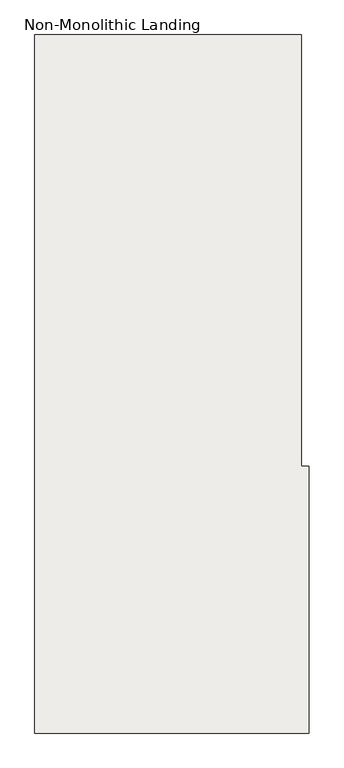
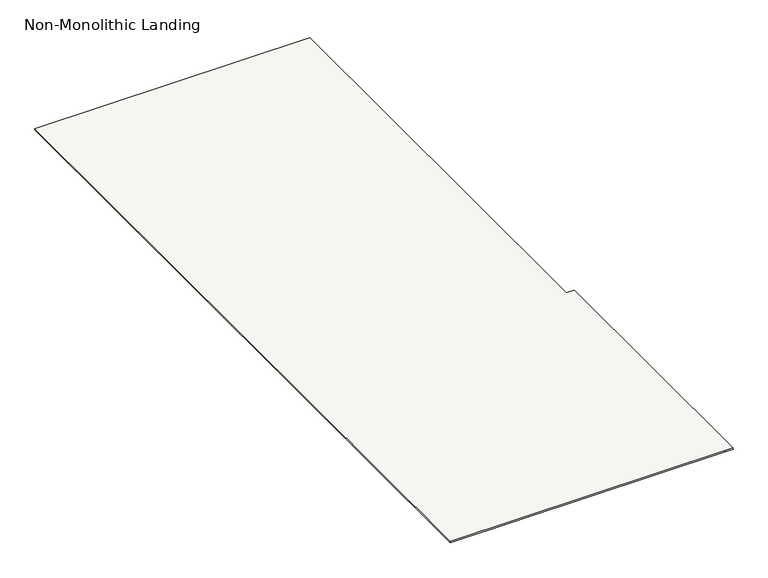
"""IFC4 building model written with IfcOpenShell, lengths in millimetres: slab geometry, Non-Monolithic Landing."""

from ifc_helpers import new_model, si_unit, origin, place, context, project, spatial, faceted_brep, source, transform, mapped, element, save


def non_monolithic_landing_19b82363(model_context):
    return source(origin(), model_context, "Body", "Brep", [
        faceted_brep([(13356.0599092, 10295.4345331, 24235.2941176), (13356.9099092, 10295.4345331, 24229.2941176), (13356.9099092, 11395.4345331, 24229.2941176), (13356.0599092, 11395.4345331, 24235.2941176), (13325.0, 13175.4345331, 24235.2941176), (12225.0, 13175.4345331, 24235.2941176), (12225.0, 10295.4345331, 24235.2941176), (13325.0, 10295.4345331, 24235.2941176), (13325.0, 11395.4345331, 24235.2941176), (13325.0, 12075.4345331, 24235.2941176), (12225.0, 10295.4345331, 24229.2941176), (12225.0, 13175.4345331, 24229.2941176), (13324.15, 13175.4345331, 24229.2941176), (13324.15, 12075.4345331, 24229.2941176), (13325.0, 12075.4345331, 24229.2941176), (13325.0, 11395.4345331, 24229.2941176), (13325.0, 10295.4345331, 24229.2941176)], [[[0, 1, 2, 3]], [[4, 5, 6, 7, 0, 3, 8, 9]], [[10, 11, 12, 13, 14, 15, 2, 1, 16]], [[9, 8, 15, 14]], [[0, 7, 16, 1]], [[7, 6, 10, 16]], [[6, 5, 11, 10]], [[5, 4, 12, 11]], [[13, 9, 14]], [[9, 13, 12, 4]], [[8, 3, 2, 15]]]),
    ])


if __name__ == "__main__":
    model = new_model("IFC4")
    model_context = context("Model", 3, world=origin())
    ifc_project = project(units=[si_unit("LENGTHUNIT", "METRE", prefix="MILLI")], contexts=[model_context])
    site = spatial("IfcSite", under=ifc_project)
    building = spatial("IfcBuilding", under=site)
    placement = place(None, origin())
    non_monolithic_landing_shape = non_monolithic_landing_19b82363(model_context)
    element("IfcSlab", 1, ObjectType="Non-Monolithic Landing", at=placement, inside=building, context=model_context, shape_type="MappedRepresentation", body=[
        mapped(non_monolithic_landing_shape, transform((0.0, 0.0, 0.0), x_axis=(1.0, 0.0, 0.0), y_axis=(0.0, 1.0, 0.0), z_axis=(0.0, 0.0, 1.0))),
    ])
    save(model, "model.ifc")

# Revit data of these elements
# Element 1 (IfcSlab, "Non-Monolithic Landing")
#   Materials on its faces: "Steel, Paint Finish, Dark Gray"
# Materials
#   "Steel, Paint Finish, Dark Gray": class "Metal", colour RGB 89 89 89, transparency 0, Description = "Steel, paint finish, dark gray, glossy", Cost = 0
